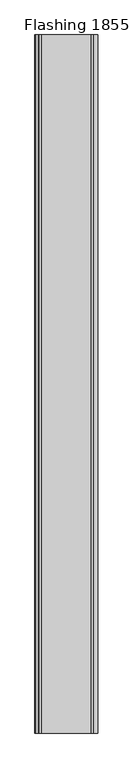
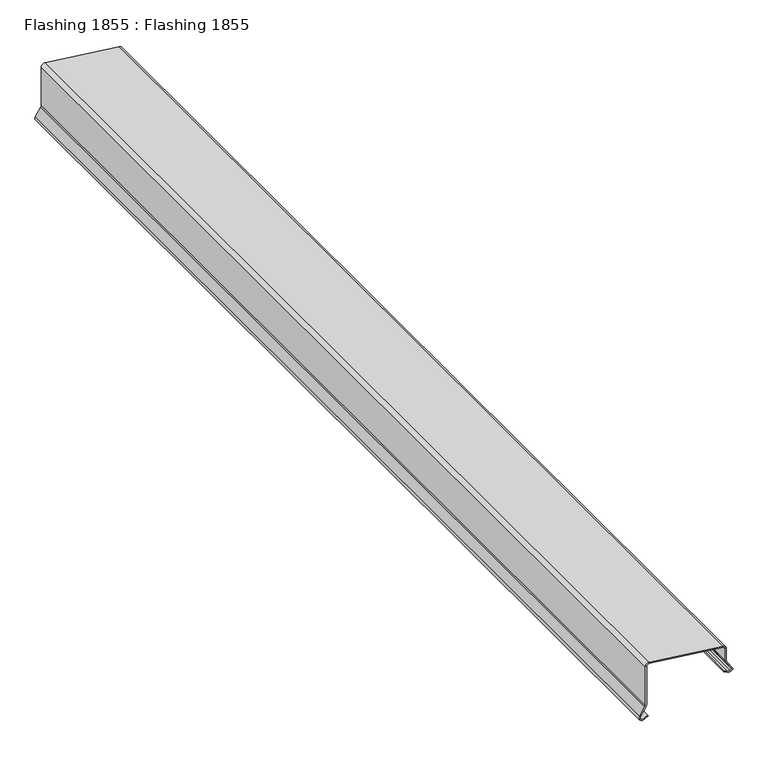
"""IFC4 building model written with IfcOpenShell, lengths in millimetres: proxy geometry, Flashing 1855 : Flashing 1855."""

from ifc_helpers import new_model, si_unit, point, frame, frame_2d, origin, place, context, project, spatial, polyline, circle_curve, trimmed, segment, composite_curve, outline, extrude, source, transform, mapped, element, save


def flashing_1855_flashing_1855_d6e76b17(model_context):
    return source(origin(), model_context, "Body", "SweptSolid", [
        extrude(outline(composite_curve([segment(trimmed(circle_curve(frame_2d((40133.2517994, -9767.0036771)), 6.35), [point((40127.5360053, -9769.7699376))], [point((40127.867313, -9763.6376994))], False, "CARTESIAN"), True, "CONTINUOUS"), segment(polyline([(40127.867313, -9763.6376994), (40130.8867187, -9758.8076172), (40149.4789842, -9770.8014653)]), True, "CONTINUOUS"), segment(trimmed(circle_curve(frame_2d((40152.9212544, -9765.4654297)), 6.35), [point((40149.4789842, -9770.8014653))], [point((40152.9212544, -9771.8154297))], True, "CARTESIAN"), True, "CONTINUOUS"), segment(polyline([(40152.9212544, -9771.8154297), (40176.1640916, -9771.8154297)]), True, "CONTINUOUS"), segment(trimmed(circle_curve(frame_2d((40176.1640916, -9778.1654297)), 6.35), [point((40176.1640916, -9771.8154297))], [point((40182.4677067, -9777.3993118))], False, "CARTESIAN"), True, "CONTINUOUS"), segment(polyline([(40182.4677067, -9777.3993118), (40199.6976336, -9919.1670852)]), True, "CONTINUOUS"), segment(trimmed(circle_curve(frame_2d((40193.3940184, -9919.9332031)), 6.35), [point((40199.6976336, -9919.1670852))], [point((40193.3940184, -9926.2832031))], False, "CARTESIAN"), True, "CONTINUOUS"), segment(polyline([(40193.3940184, -9926.2832031), (40116.1659228, -9926.2832031)]), True, "CONTINUOUS"), segment(trimmed(circle_curve(frame_2d((40116.1659228, -9932.6332031)), 6.35), [point((40116.1659228, -9926.2832031))], [point((40112.7319037, -9927.2918538))], True, "CARTESIAN"), True, "CONTINUOUS"), segment(polyline([(40112.7319037, -9927.2918538), (40096.8914441, -9937.4758802)]), True, "CONTINUOUS"), segment(trimmed(circle_curve(frame_2d((40093.4574249, -9932.1345309)), 6.35), [point((40096.8914441, -9937.4758802))], [point((40088.1090015, -9935.5575219))], False, "CARTESIAN"), True, "CONTINUOUS"), segment(polyline([(40088.1090015, -9935.5575219), (40086.3359375, -9932.7871094), (40092.1875, -9921.0800781), (40093.9764738, -9921.9742665), (40088.63264, -9932.6655014), (40089.7935443, -9934.4794145)]), True, "CONTINUOUS"), segment(trimmed(circle_curve(frame_2d((40093.4574249, -9932.1345309)), 4.35), [point((40089.7935443, -9934.4794145))], [point((40095.8098632, -9935.7935655))], True, "CARTESIAN"), True, "CONTINUOUS"), segment(polyline([(40095.8098632, -9935.7935655), (40111.6503228, -9925.6095391)]), True, "CONTINUOUS"), segment(trimmed(circle_curve(frame_2d((40116.1659228, -9932.6332031)), 8.35), [point((40111.6503228, -9925.6095391))], [point((40116.1659228, -9924.2832031))], False, "CARTESIAN"), True, "CONTINUOUS"), segment(polyline([(40116.1659228, -9924.2832031), (40193.3940184, -9924.2832031)]), True, "CONTINUOUS"), segment(trimmed(circle_curve(frame_2d((40193.3940184, -9919.9332031)), 4.35), [point((40193.3940184, -9924.2832031))], [point((40197.712243, -9919.4083822))], True, "CARTESIAN"), True, "CONTINUOUS"), segment(polyline([(40197.712243, -9919.4083822), (40180.4823161, -9777.6406088)]), True, "CONTINUOUS"), segment(trimmed(circle_curve(frame_2d((40176.1640916, -9778.1654297)), 4.35), [point((40180.4823161, -9777.6406088))], [point((40176.1640916, -9773.8154297))], True, "CARTESIAN"), True, "CONTINUOUS"), segment(polyline([(40176.1640916, -9773.8154297), (40152.9212544, -9773.8154297)]), True, "CONTINUOUS"), segment(trimmed(circle_curve(frame_2d((40152.9212544, -9765.4654297)), 8.35), [point((40152.9212544, -9773.8154297))], [point((40148.3948046, -9772.4821064))], False, "CARTESIAN"), True, "CONTINUOUS"), segment(polyline([(40148.3948046, -9772.4821064), (40131.5072723, -9761.5879796), (40129.5632143, -9764.6978498)]), True, "CONTINUOUS"), segment(trimmed(circle_curve(frame_2d((40133.2517994, -9767.0036771)), 4.35), [point((40129.5632143, -9764.6978498))], [point((40129.3362554, -9768.8986745))], True, "CARTESIAN"), True, "CONTINUOUS"), segment(polyline([(40129.3362554, -9768.8986745), (40132.6869689, -9775.8220962), (40130.8867187, -9776.6933594), (40127.5360053, -9769.7699376)]), True, "CONTINUOUS")], self_intersect=False)), frame((0.0, 7982.1531721, 0.0), z_axis=(0.0, 1.0, 0.0), x_axis=(0.0, 0.0, 1.0)), (0.0, 0.0, 1.0), 2000.0),
    ])


if __name__ == "__main__":
    model = new_model("IFC4")
    model_context = context("Model", 3, world=origin())
    ifc_project = project(units=[si_unit("LENGTHUNIT", "METRE", prefix="MILLI")], contexts=[model_context])
    site = spatial("IfcSite", under=ifc_project)
    building = spatial("IfcBuilding", under=site)
    placement = place(None, origin())
    flashing_1855_flashing_1855_shape = flashing_1855_flashing_1855_d6e76b17(model_context)
    element("IfcBuildingElementProxy", 1, Name="Flashing 1855 : Flashing 1855", ObjectType="Flashing 1855 : Flashing 1855", at=placement, inside=building, context=model_context, shape_type="MappedRepresentation", body=[
        mapped(flashing_1855_flashing_1855_shape, transform((0.0, 0.0, 0.0), x_axis=(1.0, 0.0, 0.0), y_axis=(0.0, 1.0, 0.0), z_axis=(0.0, 0.0, 1.0))),
    ])
    save(model, "model.ifc")

# Revit data of these elements
# Type "Flashing 1855 : Flashing 1855"
#   NameOverride = "Flashing"
# Element 1 (IfcBuildingElementProxy, "Flashing 1855 : Flashing 1855")
#   Materials on its faces: "METAL COPING"
# Materials
#   "METAL COPING": class "Unassigned", colour RGB 128 128 128, transparency 0
